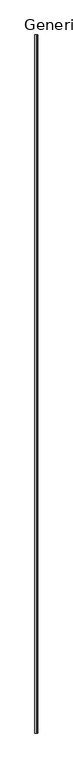
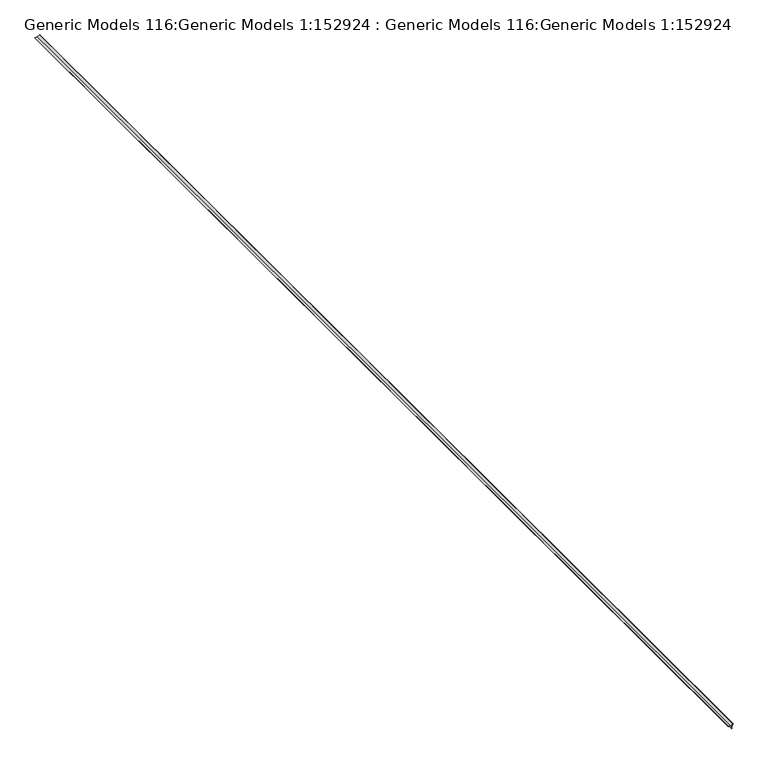
"""IFC4 building model written with IfcOpenShell, lengths in millimetres: proxy geometry, Generic Models 116:Generic Models 1:152924 : Generic Models 116:Generic Models 1:152924."""

from ifc_helpers import new_model, si_unit, point, frame, frame_2d, origin, place, context, project, spatial, polyline, circle_curve, trimmed, segment, composite_curve, outline, extrude, source, transform, mapped, element, save


def generic_models_116_generic_models_1_152924_generic_models_cc373daa(model_context):
    return source(origin(), model_context, "Body", "SweptSolid", [
        extrude(outline(composite_curve([segment(trimmed(circle_curve(frame_2d((3804.0592495, 7259.6690004)), 1.4342127), [point((3803.4040944, 7260.9448287))], [point((3805.3350778, 7259.0138453))], False, "CARTESIAN"), True, "CONTINUOUS"), segment(polyline([(3805.3350778, 7259.0138453), (3785.8084622, 7220.9883307), (3785.8084622, 7182.8883307), (3784.5384622, 7182.8883307), (3784.5384622, 7221.2953544), (3804.4387018, 7260.0484527), (3765.6856036, 7240.1482131), (3727.2785798, 7240.1482131), (3727.2785798, 7241.4182131), (3765.3785798, 7241.4182131), (3803.4040944, 7260.9448287)]), True, "CONTINUOUS")], self_intersect=False)), frame((0.0, -6877.9974793, 0.0), z_axis=(0.0, 1.0, 0.0), x_axis=(0.0, 0.0, 1.0)), (0.0, 0.0, 1.0), 19050.0),
    ])


if __name__ == "__main__":
    model = new_model("IFC4")
    model_context = context("Model", 3, world=origin())
    ifc_project = project(units=[si_unit("LENGTHUNIT", "METRE", prefix="MILLI")], contexts=[model_context])
    site = spatial("IfcSite", under=ifc_project)
    building = spatial("IfcBuilding", under=site)
    placement = place(None, origin())
    generic_models_116_generic_models_1_152924_generic_models_shape = generic_models_116_generic_models_1_152924_generic_models_cc373daa(model_context)
    element("IfcBuildingElementProxy", 1, Name="Generic Models 116:Generic Models 1:152924 : Generic Models 116:Generic Models 1:152924", ObjectType="Generic Models 116:Generic Models 1:152924 : Generic Models 116:Generic Models 1:152924", at=placement, inside=building, context=model_context, shape_type="MappedRepresentation", body=[
        mapped(generic_models_116_generic_models_1_152924_generic_models_shape, transform((0.0, 0.0, 0.0), x_axis=(1.0, 0.0, 0.0), y_axis=(0.0, 1.0, 0.0), z_axis=(0.0, 0.0, 1.0))),
    ])
    save(model, "model.ifc")

# Revit data of these elements
# Type "Generic Models 116:Generic Models 1:152924 : Generic Models 116:Generic Models 1:152924"
#   NameOverride = "Generic Models 116:Generic Models 1:152924"
#   ObjectTypeOverride = "Generic Models 116:Generic Models 1"
#   Reference = "Generic Models 1"
#   Category = "Generic Models"
#   Tag = "152924"
# Element 1 (IfcBuildingElementProxy, "Generic Models 116:Generic Models 1:152924 : Generic Models 116:Generic Models 1:152924")
#   Materials on its faces: "_CONTINUOUS 16 GA. COPPER CORNER BEAD 558"
# Materials
#   "_CONTINUOUS 16 GA. COPPER CORNER BEAD 558": class "Unassigned", colour RGB 253 192 103, transparency 0
